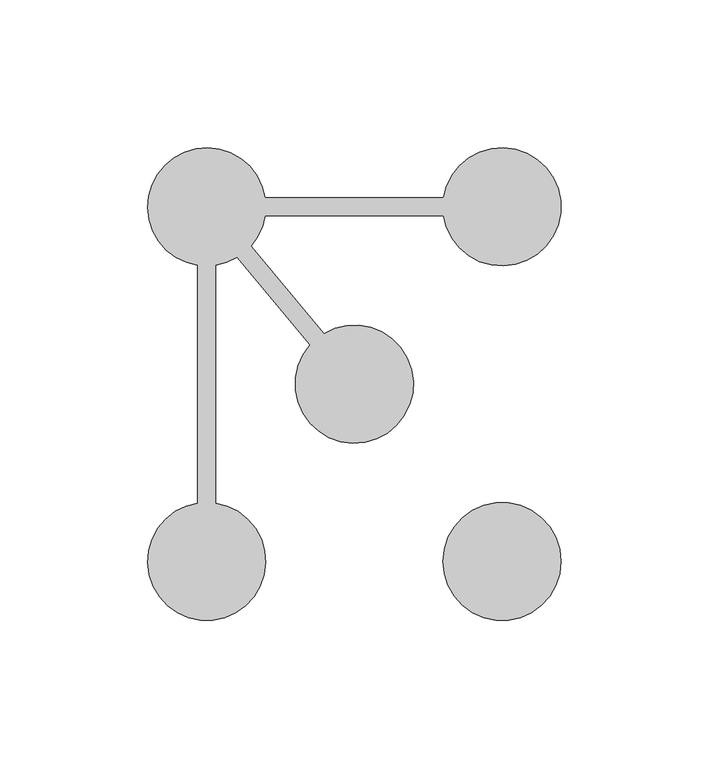
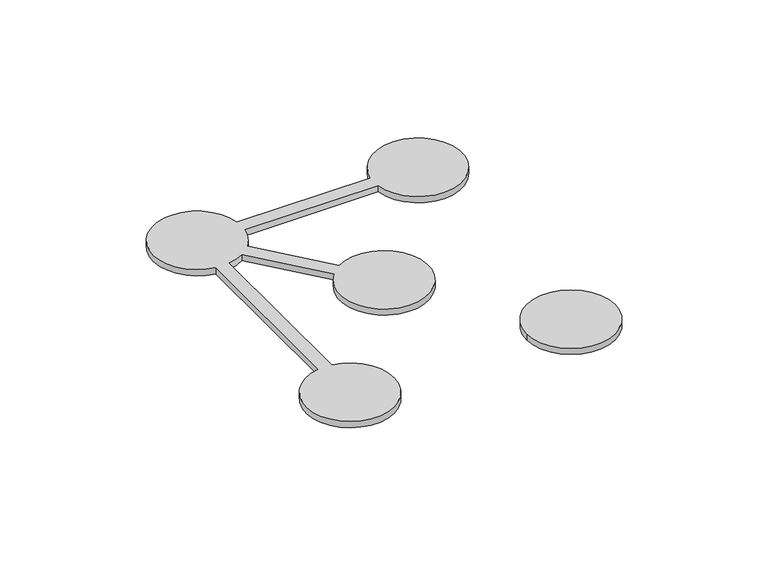
"""IFC4 building model written with IfcOpenShell, lengths in millimetres: proxy geometry, TSP Footlight points : TSP Footlight points."""

from ifc_helpers import new_model, si_unit, point, frame_2d, origin, origin_with_axes, origin_2d, place, context, project, spatial, polyline, circle_curve, trimmed, segment, composite_curve, outline, extrude, source, transform, mapped, element, save


def electrical_fixtures_37d56e3e(model_context):
    return source(origin(), model_context, "Body", "SweptSolid", [
        extrude(outline(composite_curve([segment(trimmed(circle_curve(frame_2d((50.0, -60.0)), 20.0), [point((70.0, -60.0))], [point((30.0, -60.0))], False, "CARTESIAN"), True, "CONTINUOUS"), segment(trimmed(circle_curve(frame_2d((50.0, -60.0)), 20.0), [point((30.0, -60.0))], [point((70.0, -60.0))], False, "CARTESIAN"), True, "CONTINUOUS")], self_intersect=False)), origin_with_axes(), (0.0, 0.0, 1.0), 3.0),
        extrude(outline(composite_curve([segment(trimmed(circle_curve(origin_2d(), 20.0), [point((-10.3541632, 17.1111456))], [point((-14.9634909, 13.2700392))], False, "CARTESIAN"), True, "CONTINUOUS"), segment(polyline([(-14.9634909, 13.2700392), (-39.6458368, 42.8888544)]), True, "CONTINUOUS"), segment(trimmed(circle_curve(frame_2d((-50.0, 60.0)), 20.0), [point((-39.6458368, 42.8888544))], [point((-47.0, 40.2262801))], False, "CARTESIAN"), True, "CONTINUOUS"), segment(polyline([(-47.0, 40.2262801), (-47.0, -40.2262801)]), True, "CONTINUOUS"), segment(trimmed(circle_curve(frame_2d((-50.0, -60.0)), 20.0), [point((-47.0, -40.2262801))], [point((-53.0, -40.2262801))], False, "CARTESIAN"), True, "CONTINUOUS"), segment(polyline([(-53.0, -40.2262801), (-53.0, 40.2262801)]), True, "CONTINUOUS"), segment(trimmed(circle_curve(frame_2d((-50.0, 60.0)), 20.0), [point((-53.0, 40.2262801))], [point((-30.2262801, 63.0))], False, "CARTESIAN"), True, "CONTINUOUS"), segment(polyline([(-30.2262801, 63.0), (30.2262801, 63.0)]), True, "CONTINUOUS"), segment(trimmed(circle_curve(frame_2d((50.0, 60.0)), 20.0), [point((30.2262801, 63.0))], [point((30.2262801, 57.0))], False, "CARTESIAN"), True, "CONTINUOUS"), segment(polyline([(30.2262801, 57.0), (-30.2262801, 57.0)]), True, "CONTINUOUS"), segment(trimmed(circle_curve(frame_2d((-50.0, 60.0)), 20.0), [point((-30.2262801, 57.0))], [point((-35.0365091, 46.7299608))], False, "CARTESIAN"), True, "CONTINUOUS"), segment(polyline([(-35.0365091, 46.7299608), (-10.3541632, 17.1111456)]), True, "CONTINUOUS")], self_intersect=False)), origin_with_axes(), (0.0, 0.0, 1.0), 3.0),
    ])


if __name__ == "__main__":
    model = new_model("IFC4")
    model_context = context("Model", 3, world=origin())
    ifc_project = project(units=[si_unit("LENGTHUNIT", "METRE", prefix="MILLI")], contexts=[model_context])
    site = spatial("IfcSite", under=ifc_project)
    building = spatial("IfcBuilding", under=site)
    placement = place(None, origin())
    electrical_fixtures_shape = electrical_fixtures_37d56e3e(model_context)
    element("IfcBuildingElementProxy", 1, Name="TSP Footlight points : TSP Footlight points", ObjectType="TSP Footlight points : TSP Footlight points", at=placement, inside=building, context=model_context, shape_type="MappedRepresentation", body=[
        mapped(electrical_fixtures_shape, transform((0.0, 0.0, 0.0), x_axis=(1.0, 0.0, 0.0), y_axis=(0.0, 1.0, 0.0), z_axis=(0.0, 0.0, 1.0))),
    ])
    save(model, "model.ifc")

# Revit data of these elements
# Type "TSP Footlight points : TSP Footlight points"
#   Model = "TSP_ELECLVFLP"
#   Default Elevation = 0
# Element 1 (IfcBuildingElementProxy, "TSP Footlight points : TSP Footlight points")
#   Materials on its faces: "Plastic, Opaque Black"
# Materials
#   "Plastic, Opaque Black": class "Plastic", colour RGB 0 0 0, transparency 0.7, Description = "Plastic, generic, opaque black", Cost = 0
